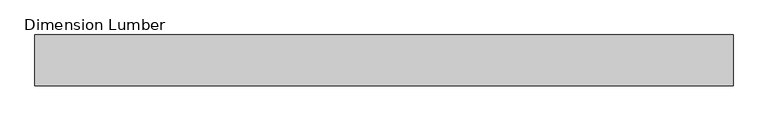
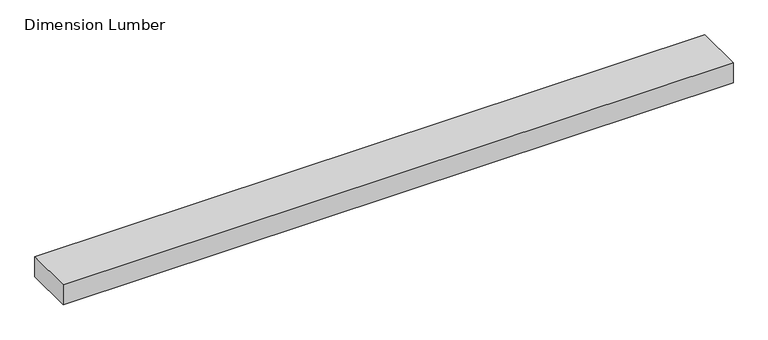
"""IFC4 building model written with IfcOpenShell, lengths in millimetres: beam geometry, Dimension Lumber : Opening Plate 2*4 Exterior."""

import ifcopenshell
import ifcopenshell.guid

model = None  # the IFC model being written
_history = None  # IfcOwnerHistory: only IFC2X3 demands one
_inside = {}  # id of a spatial element -> (the spatial element, [elements in it])
_under = {}  # id of a project, library or spatial element -> (it, [spatial elements below it])
_declared = {}  # id of a project -> (the project, [libraries it declares])
_typed = {}  # id of a type object -> (the type object, [elements of that type])
_made_of = {}  # id of a material, layer set ... -> (it, [elements and type objects made of it])


def new_model(schema):
    """Start an empty IFC model of exactly this schema.

    Asked for "IFC4X3", IfcOpenShell would pick the latest addendum, in which some entities
    have other attributes; the version numbers below select the first issue.
    IFC2X3 requires an IfcOwnerHistory on every rooted entity: one is made here for all.
    """
    global model, _history
    if schema == "IFC4X3":
        model = ifcopenshell.file(schema_version=(4, 3, 0, 0))
    else:
        model = ifcopenshell.file(schema=schema)
    _inside.clear()
    _under.clear()
    _declared.clear()
    _typed.clear()
    _made_of.clear()
    _history = None
    if model.schema == "IFC2X3":
        org = make("IfcOrganization", Name="unknown")
        user = make(
            "IfcPersonAndOrganization",
            ThePerson=make("IfcPerson", FamilyName="unknown"),
            TheOrganization=org,
        )
        app = make(
            "IfcApplication",
            ApplicationDeveloper=org,
            Version="unknown",
            ApplicationFullName="unknown",
            ApplicationIdentifier="unknown",
        )
        _history = make(
            "IfcOwnerHistory",
            OwningUser=user,
            OwningApplication=app,
            ChangeAction="ADDED",
            CreationDate=0,
        )
    return model


def make(cls, **values):
    """One entity of the class cls with the attributes given. An attribute that is None is left unset."""
    return model.create_entity(
        cls, **{name: value for name, value in values.items() if value is not None}
    )


def rooted(cls, **values):
    """An entity with a GlobalId (a new one), such as an element, a storey or a relation."""
    return make(cls, GlobalId=ifcopenshell.guid.new(), OwnerHistory=_history, **values)


def si_unit(unit_type, name, prefix=None):
    """IfcSIUnit, for example si_unit("LENGTHUNIT", "METRE", prefix="MILLI")."""
    return make("IfcSIUnit", UnitType=unit_type, Prefix=prefix, Name=name)


def assignment(units):
    """IfcUnitAssignment: the units of a project."""
    return None if units is None else make("IfcUnitAssignment", Units=units)


def point(xyz):
    """IfcCartesianPoint."""
    return None if xyz is None else make("IfcCartesianPoint", Coordinates=xyz)


def direction(xyz):
    """IfcDirection."""
    return None if xyz is None else make("IfcDirection", DirectionRatios=xyz)


def frame(location, z_axis=None, x_axis=None):
    """IfcAxis2Placement3D, a coordinate frame: its origin and axes. An axis left out is left unset."""
    return make(
        "IfcAxis2Placement3D",
        Location=point(location),
        Axis=direction(z_axis),
        RefDirection=direction(x_axis),
    )


def origin():
    """The frame at (0, 0, 0) with its axes left unset."""
    return frame((0.0, 0.0, 0.0))


def place(relative_to, where):
    """IfcLocalPlacement: puts the frame where relative to a parent placement (None: the world)."""
    return make(
        "IfcLocalPlacement", PlacementRelTo=relative_to, RelativePlacement=where
    )


def context(
    kind, dimensions, precision=None, world=None, true_north=None, identifier=None
):
    """IfcGeometricRepresentationContext, for example the 3D "Model" context."""
    return make(
        "IfcGeometricRepresentationContext",
        ContextIdentifier=identifier,
        ContextType=kind,
        CoordinateSpaceDimension=dimensions,
        Precision=precision,
        WorldCoordinateSystem=world,
        TrueNorth=true_north,
    )


def project(units=None, contexts=None):
    """IfcProject with its units and contexts."""
    return rooted(
        "IfcProject",
        Name="project",
        RepresentationContexts=contexts,
        UnitsInContext=assignment(units),
    )


def spatial(cls, under=None, at=None, **own):
    """A site, building, storey or space (cls), placed at a placement, below another one or the project."""
    s = rooted(cls, ObjectPlacement=at, **own)
    if under is not None:
        _under.setdefault(under.id(), (under, []))[1].append(s)
    return s


def polyline(points):
    """IfcPolyline through the points."""
    return make("IfcPolyline", Points=[point(p) for p in points])


def outline(outer, holes=None, kind="AREA"):
    """IfcArbitraryClosedProfileDef: a profile drawn as a closed curve; with holes, ...WithVoids."""
    if holes is None:
        return make("IfcArbitraryClosedProfileDef", ProfileType=kind, OuterCurve=outer)
    return make(
        "IfcArbitraryProfileDefWithVoids",
        ProfileType=kind,
        OuterCurve=outer,
        InnerCurves=holes,
    )


def extrude(swept, where, along, depth):
    """IfcExtrudedAreaSolid: the profile swept, set in the frame where, extruded along a direction by depth."""
    return make(
        "IfcExtrudedAreaSolid",
        SweptArea=swept,
        Position=where,
        ExtrudedDirection=direction(along),
        Depth=depth,
    )


def shape(context_of_items, identifier, shape_type, items):
    """IfcShapeRepresentation: the items that make up one representation, for example the "Body"."""
    return make(
        "IfcShapeRepresentation",
        ContextOfItems=context_of_items,
        RepresentationIdentifier=identifier,
        RepresentationType=shape_type,
        Items=items,
    )


def source(mapping_origin, context_of_items, identifier, shape_type, items):
    """IfcRepresentationMap: a shape defined once, which mapped items show again and again."""
    return make(
        "IfcRepresentationMap",
        MappingOrigin=mapping_origin,
        MappedRepresentation=shape(context_of_items, identifier, shape_type, items),
    )


def transform(
    local_origin,
    x_axis=None,
    y_axis=None,
    z_axis=None,
    scale=None,
    scale2=None,
    scale3=None,
    uniform=True,
):
    """IfcCartesianTransformationOperator3D, or its non-uniform kind. x_axis, y_axis, z_axis: its Axis1, 2, 3."""
    if uniform:
        return make(
            "IfcCartesianTransformationOperator3D",
            Axis1=direction(x_axis),
            Axis2=direction(y_axis),
            LocalOrigin=point(local_origin),
            Scale=scale,
            Axis3=direction(z_axis),
        )
    return make(
        "IfcCartesianTransformationOperator3DnonUniform",
        Axis1=direction(x_axis),
        Axis2=direction(y_axis),
        LocalOrigin=point(local_origin),
        Scale=scale,
        Axis3=direction(z_axis),
        Scale2=scale2,
        Scale3=scale3,
    )


def mapped(mapping_source, mapping_target):
    """IfcMappedItem: shows the shape of a source again, moved by a transform."""
    return make(
        "IfcMappedItem", MappingSource=mapping_source, MappingTarget=mapping_target
    )


def made_of(thing, what):
    """Note that an element or type object is made of a material, layer set ...; save() writes the relation."""
    if what is not None:
        _made_of.setdefault(what.id(), (what, []))[1].append(thing)
    return thing


def element(
    cls,
    number,
    at=None,
    inside=None,
    cuts=None,
    type_object=None,
    material=None,
    context=None,
    identifier="Body",
    shape_type=None,
    held_by="IfcProductDefinitionShape",
    body=None,
    shapes=None,
    **own,
):
    """One element of the class cls, such as IfcWall. Its Tag is "e" and its number.

    at: its placement. inside: the storey or other place that contains it. cuts: it is an
    opening in that element (IfcRelVoidsElement). A single representation is given by context,
    identifier, shape_type and body (its items); several are given by shapes. held_by: the class
    of the entity that holds the representations. save() writes the other relations.
    """
    e = rooted(cls, Tag="e%d" % number, ObjectPlacement=at, **own)
    if body is not None:
        shapes = [shape(context, identifier, shape_type, body)]
    if shapes is not None:
        e.Representation = make(held_by, Representations=shapes)
    if inside is not None:
        _inside.setdefault(inside.id(), (inside, []))[1].append(e)
    if cuts is not None:
        rooted(
            "IfcRelVoidsElement", RelatingBuildingElement=cuts, RelatedOpeningElement=e
        )
    if type_object is not None:
        _typed.setdefault(type_object.id(), (type_object, []))[1].append(e)
    return made_of(e, material)


def aggregate(whole, parts):
    """IfcRelAggregates: a whole, such as a stair, and the parts it consists of."""
    return rooted("IfcRelAggregates", RelatingObject=whole, RelatedObjects=parts)


def save(model, path):
    """Write the relations noted so far, then the file.

    IfcRelAggregates (storeys below a building ...), IfcRelContainedInSpatialStructure (elements
    in a storey), IfcRelDefinesByType, IfcRelAssociatesMaterial and IfcRelDeclares: one each for
    every whole, place, type object, material and project.
    """
    for whole, parts in _under.values():
        aggregate(whole, parts)
    for where, things in _inside.values():
        rooted(
            "IfcRelContainedInSpatialStructure",
            RelatedElements=things,
            RelatingStructure=where,
        )
    for kind, things in _typed.values():
        rooted("IfcRelDefinesByType", RelatedObjects=things, RelatingType=kind)
    for what, things in _made_of.values():
        rooted("IfcRelAssociatesMaterial", RelatedObjects=things, RelatingMaterial=what)
    for by, libraries in _declared.values():
        rooted("IfcRelDeclares", RelatingContext=by, RelatedDefinitions=libraries)
    model.write(path)


def dimension_lumber_37c2d9e3(model_context):
    return source(origin(), model_context, "Body", "SweptSolid", [
        extrude(outline(polyline([(609.5999994, 44.45), (609.5999994, -44.45), (-609.5999994, -44.45), (-609.5999994, 44.45), (609.5999994, 44.45)])), frame((0.0, 0.0, -19.05), z_axis=(0.0, 0.0, 1.0), x_axis=(1.0, 0.0, 0.0)), (0.0, 0.0, 1.0), 38.1),
    ])


if __name__ == "__main__":
    model = new_model("IFC4")
    model_context = context("Model", 3, world=origin())
    ifc_project = project(units=[si_unit("LENGTHUNIT", "METRE", prefix="MILLI")], contexts=[model_context])
    site = spatial("IfcSite", under=ifc_project)
    building = spatial("IfcBuilding", under=site)
    placement = place(None, origin())
    dimension_lumber_shape = dimension_lumber_37c2d9e3(model_context)
    element("IfcBeam", 1, ObjectType="Dimension Lumber : Opening Plate 2*4 Exterior", at=placement, inside=building, context=model_context, shape_type="MappedRepresentation", body=[
        mapped(dimension_lumber_shape, transform((0.0, 0.0, 0.0), x_axis=(1.0, 0.0, 0.0), y_axis=(0.0, 1.0, 0.0), z_axis=(0.0, 0.0, 1.0))),
    ])
    save(model, "model.ifc")

# Revit data of these elements
# Type "Dimension Lumber : Opening Plate 2*4 Exterior"
#   Assembly Code = "B10"
#   A = 0.0364583 SF
#   Length [instance default] = 5' - 0"
#   b = 0' - 3 1/2"
#   d = 0' - 1 1/2"
#   Structural Material [instance default] = Softwood, Lumber
# Element 1 (IfcBeam, "Dimension Lumber : Opening Plate 2*4 Exterior")
#   Structural Material = Douglas Fir #2
#   Materials on its faces: "Douglas Fir #2"
# Materials
#   "Softwood, Lumber": class "Wood", colour RGB 223 192 134, transparency 0, Description = "Pinus Echinata", Cost = 0
#   "Douglas Fir #2": class "Wood", colour RGB 223 192 134, transparency 0, Description = "Pinus Echinata", Cost = 0
